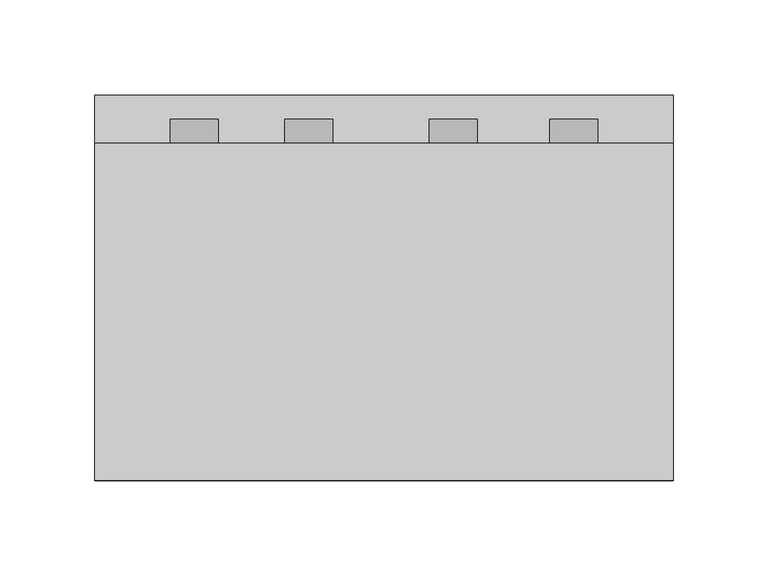
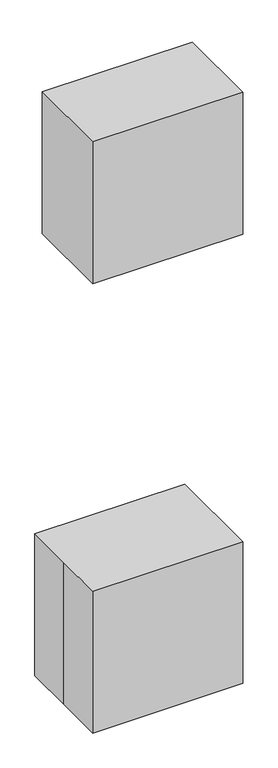
"""IFC4 building model written with IfcOpenShell, lengths in millimetres: proxy geometry, M7845 - Monitor, Physiological, Bedside, 4 Channel-mobile : M7845 - Monitor, Physiological, Bedside, 4 Channel-mobile."""

import ifcopenshell
import ifcopenshell.guid

model = None  # the IFC model being written
_history = None  # IfcOwnerHistory: only IFC2X3 demands one
_inside = {}  # id of a spatial element -> (the spatial element, [elements in it])
_under = {}  # id of a project, library or spatial element -> (it, [spatial elements below it])
_declared = {}  # id of a project -> (the project, [libraries it declares])
_typed = {}  # id of a type object -> (the type object, [elements of that type])
_made_of = {}  # id of a material, layer set ... -> (it, [elements and type objects made of it])


def new_model(schema):
    """Start an empty IFC model of exactly this schema.

    Asked for "IFC4X3", IfcOpenShell would pick the latest addendum, in which some entities
    have other attributes; the version numbers below select the first issue.
    IFC2X3 requires an IfcOwnerHistory on every rooted entity: one is made here for all.
    """
    global model, _history
    if schema == "IFC4X3":
        model = ifcopenshell.file(schema_version=(4, 3, 0, 0))
    else:
        model = ifcopenshell.file(schema=schema)
    _inside.clear()
    _under.clear()
    _declared.clear()
    _typed.clear()
    _made_of.clear()
    _history = None
    if model.schema == "IFC2X3":
        org = make("IfcOrganization", Name="unknown")
        user = make(
            "IfcPersonAndOrganization",
            ThePerson=make("IfcPerson", FamilyName="unknown"),
            TheOrganization=org,
        )
        app = make(
            "IfcApplication",
            ApplicationDeveloper=org,
            Version="unknown",
            ApplicationFullName="unknown",
            ApplicationIdentifier="unknown",
        )
        _history = make(
            "IfcOwnerHistory",
            OwningUser=user,
            OwningApplication=app,
            ChangeAction="ADDED",
            CreationDate=0,
        )
    return model


def make(cls, **values):
    """One entity of the class cls with the attributes given. An attribute that is None is left unset."""
    return model.create_entity(
        cls, **{name: value for name, value in values.items() if value is not None}
    )


def rooted(cls, **values):
    """An entity with a GlobalId (a new one), such as an element, a storey or a relation."""
    return make(cls, GlobalId=ifcopenshell.guid.new(), OwnerHistory=_history, **values)


def si_unit(unit_type, name, prefix=None):
    """IfcSIUnit, for example si_unit("LENGTHUNIT", "METRE", prefix="MILLI")."""
    return make("IfcSIUnit", UnitType=unit_type, Prefix=prefix, Name=name)


def assignment(units):
    """IfcUnitAssignment: the units of a project."""
    return None if units is None else make("IfcUnitAssignment", Units=units)


def point(xyz):
    """IfcCartesianPoint."""
    return None if xyz is None else make("IfcCartesianPoint", Coordinates=xyz)


def direction(xyz):
    """IfcDirection."""
    return None if xyz is None else make("IfcDirection", DirectionRatios=xyz)


def frame(location, z_axis=None, x_axis=None):
    """IfcAxis2Placement3D, a coordinate frame: its origin and axes. An axis left out is left unset."""
    return make(
        "IfcAxis2Placement3D",
        Location=point(location),
        Axis=direction(z_axis),
        RefDirection=direction(x_axis),
    )


def frame_2d(location, x_axis=None):
    """IfcAxis2Placement2D, a coordinate frame in the plane: its origin and x axis."""
    return make(
        "IfcAxis2Placement2D", Location=point(location), RefDirection=direction(x_axis)
    )


def origin():
    """The frame at (0, 0, 0) with its axes left unset."""
    return frame((0.0, 0.0, 0.0))


def origin_with_axes():
    """The frame at (0, 0, 0) with the z axis (0, 0, 1) and the x axis (1, 0, 0) written out."""
    return frame((0.0, 0.0, 0.0), z_axis=(0.0, 0.0, 1.0), x_axis=(1.0, 0.0, 0.0))


def place(relative_to, where):
    """IfcLocalPlacement: puts the frame where relative to a parent placement (None: the world)."""
    return make(
        "IfcLocalPlacement", PlacementRelTo=relative_to, RelativePlacement=where
    )


def context(
    kind, dimensions, precision=None, world=None, true_north=None, identifier=None
):
    """IfcGeometricRepresentationContext, for example the 3D "Model" context."""
    return make(
        "IfcGeometricRepresentationContext",
        ContextIdentifier=identifier,
        ContextType=kind,
        CoordinateSpaceDimension=dimensions,
        Precision=precision,
        WorldCoordinateSystem=world,
        TrueNorth=true_north,
    )


def project(units=None, contexts=None):
    """IfcProject with its units and contexts."""
    return rooted(
        "IfcProject",
        Name="project",
        RepresentationContexts=contexts,
        UnitsInContext=assignment(units),
    )


def spatial(cls, under=None, at=None, **own):
    """A site, building, storey or space (cls), placed at a placement, below another one or the project."""
    s = rooted(cls, ObjectPlacement=at, **own)
    if under is not None:
        _under.setdefault(under.id(), (under, []))[1].append(s)
    return s


def polyline(points):
    """IfcPolyline through the points."""
    return make("IfcPolyline", Points=[point(p) for p in points])


def circle_curve(where, radius):
    """IfcCircle in the frame where."""
    return make("IfcCircle", Position=where, Radius=radius)


def trimmed(basis, trim1, trim2, sense, master):
    """IfcTrimmedCurve: the piece of a basis curve between two trims."""
    return make(
        "IfcTrimmedCurve",
        BasisCurve=basis,
        Trim1=trim1,
        Trim2=trim2,
        SenseAgreement=sense,
        MasterRepresentation=master,
    )


def segment(curve, same_sense, transition):
    """IfcCompositeCurveSegment."""
    return make(
        "IfcCompositeCurveSegment",
        Transition=transition,
        SameSense=same_sense,
        ParentCurve=curve,
    )


def composite_curve(segments, self_intersect=None):
    """IfcCompositeCurve: segments joined end to end."""
    return make("IfcCompositeCurve", Segments=segments, SelfIntersect=self_intersect)


def outline(outer, holes=None, kind="AREA"):
    """IfcArbitraryClosedProfileDef: a profile drawn as a closed curve; with holes, ...WithVoids."""
    if holes is None:
        return make("IfcArbitraryClosedProfileDef", ProfileType=kind, OuterCurve=outer)
    return make(
        "IfcArbitraryProfileDefWithVoids",
        ProfileType=kind,
        OuterCurve=outer,
        InnerCurves=holes,
    )


def extrude(swept, where, along, depth):
    """IfcExtrudedAreaSolid: the profile swept, set in the frame where, extruded along a direction by depth."""
    return make(
        "IfcExtrudedAreaSolid",
        SweptArea=swept,
        Position=where,
        ExtrudedDirection=direction(along),
        Depth=depth,
    )


def faces_of(points, faces, orient=None, outer=None):
    """IfcFace entities. A face is a list of loops; a loop is a list of indices into points, from 0.

    orient and outer hold one flag for each loop. By default every Orientation is true, the
    first loop of a face is its IfcFaceOuterBound and the others are IfcFaceBound.
    """
    made = []
    for i, loops in enumerate(faces):
        bounds = []
        for j, loop in enumerate(loops):
            is_outer = j == 0 if outer is None else outer[i][j]
            bounds.append(
                make(
                    "IfcFaceOuterBound" if is_outer else "IfcFaceBound",
                    Bound=make("IfcPolyLoop", Polygon=[points[k] for k in loop]),
                    Orientation=True if orient is None else orient[i][j],
                )
            )
        made.append(make("IfcFace", Bounds=bounds))
    return made


def faceted_brep(points, faces, orient=None, outer=None, voids=None):
    """IfcFacetedBrep: a solid bounded by flat faces; with voids (closed shells), ...WithVoids."""
    shared = [point(p) for p in points]
    hull = make("IfcClosedShell", CfsFaces=faces_of(shared, faces, orient, outer))
    if voids is None:
        return make("IfcFacetedBrep", Outer=hull)
    return make(
        "IfcFacetedBrepWithVoids",
        Outer=hull,
        Voids=[
            make(cls, CfsFaces=faces_of(shared, fs, o, b)) for cls, fs, o, b in voids
        ],
    )


def shape(context_of_items, identifier, shape_type, items):
    """IfcShapeRepresentation: the items that make up one representation, for example the "Body"."""
    return make(
        "IfcShapeRepresentation",
        ContextOfItems=context_of_items,
        RepresentationIdentifier=identifier,
        RepresentationType=shape_type,
        Items=items,
    )


def source(mapping_origin, context_of_items, identifier, shape_type, items):
    """IfcRepresentationMap: a shape defined once, which mapped items show again and again."""
    return make(
        "IfcRepresentationMap",
        MappingOrigin=mapping_origin,
        MappedRepresentation=shape(context_of_items, identifier, shape_type, items),
    )


def transform(
    local_origin,
    x_axis=None,
    y_axis=None,
    z_axis=None,
    scale=None,
    scale2=None,
    scale3=None,
    uniform=True,
):
    """IfcCartesianTransformationOperator3D, or its non-uniform kind. x_axis, y_axis, z_axis: its Axis1, 2, 3."""
    if uniform:
        return make(
            "IfcCartesianTransformationOperator3D",
            Axis1=direction(x_axis),
            Axis2=direction(y_axis),
            LocalOrigin=point(local_origin),
            Scale=scale,
            Axis3=direction(z_axis),
        )
    return make(
        "IfcCartesianTransformationOperator3DnonUniform",
        Axis1=direction(x_axis),
        Axis2=direction(y_axis),
        LocalOrigin=point(local_origin),
        Scale=scale,
        Axis3=direction(z_axis),
        Scale2=scale2,
        Scale3=scale3,
    )


def mapped(mapping_source, mapping_target):
    """IfcMappedItem: shows the shape of a source again, moved by a transform."""
    return make(
        "IfcMappedItem", MappingSource=mapping_source, MappingTarget=mapping_target
    )


def made_of(thing, what):
    """Note that an element or type object is made of a material, layer set ...; save() writes the relation."""
    if what is not None:
        _made_of.setdefault(what.id(), (what, []))[1].append(thing)
    return thing


def element(
    cls,
    number,
    at=None,
    inside=None,
    cuts=None,
    type_object=None,
    material=None,
    context=None,
    identifier="Body",
    shape_type=None,
    held_by="IfcProductDefinitionShape",
    body=None,
    shapes=None,
    **own,
):
    """One element of the class cls, such as IfcWall. Its Tag is "e" and its number.

    at: its placement. inside: the storey or other place that contains it. cuts: it is an
    opening in that element (IfcRelVoidsElement). A single representation is given by context,
    identifier, shape_type and body (its items); several are given by shapes. held_by: the class
    of the entity that holds the representations. save() writes the other relations.
    """
    e = rooted(cls, Tag="e%d" % number, ObjectPlacement=at, **own)
    if body is not None:
        shapes = [shape(context, identifier, shape_type, body)]
    if shapes is not None:
        e.Representation = make(held_by, Representations=shapes)
    if inside is not None:
        _inside.setdefault(inside.id(), (inside, []))[1].append(e)
    if cuts is not None:
        rooted(
            "IfcRelVoidsElement", RelatingBuildingElement=cuts, RelatedOpeningElement=e
        )
    if type_object is not None:
        _typed.setdefault(type_object.id(), (type_object, []))[1].append(e)
    return made_of(e, material)


def aggregate(whole, parts):
    """IfcRelAggregates: a whole, such as a stair, and the parts it consists of."""
    return rooted("IfcRelAggregates", RelatingObject=whole, RelatedObjects=parts)


def save(model, path):
    """Write the relations noted so far, then the file.

    IfcRelAggregates (storeys below a building ...), IfcRelContainedInSpatialStructure (elements
    in a storey), IfcRelDefinesByType, IfcRelAssociatesMaterial and IfcRelDeclares: one each for
    every whole, place, type object, material and project.
    """
    for whole, parts in _under.values():
        aggregate(whole, parts)
    for where, things in _inside.values():
        rooted(
            "IfcRelContainedInSpatialStructure",
            RelatedElements=things,
            RelatingStructure=where,
        )
    for kind, things in _typed.values():
        rooted("IfcRelDefinesByType", RelatedObjects=things, RelatingType=kind)
    for what, things in _made_of.values():
        rooted("IfcRelAssociatesMaterial", RelatedObjects=things, RelatingMaterial=what)
    for by, libraries in _declared.values():
        rooted("IfcRelDeclares", RelatingContext=by, RelatedDefinitions=libraries)
    model.write(path)


def specialty_equipment_01cb5a5e(model_context):
    return source(origin(), model_context, "Body", "SolidModel", [
        extrude(outline(composite_curve([segment(trimmed(circle_curve(frame_2d((1006.3587525, 100.0366492)), 12.7), [point((1006.3587525, 112.7366492))], [point((1006.3587525, 87.3366492))], False, "CARTESIAN"), True, "CONTINUOUS"), segment(trimmed(circle_curve(frame_2d((1006.3587525, 100.0366492)), 12.7), [point((1006.3587525, 87.3366492))], [point((1006.3587525, 112.7366492))], False, "CARTESIAN"), True, "CONTINUOUS")], self_intersect=False)), frame((0.0, 76.2, 0.0), z_axis=(0.0, 1.0, 0.0), x_axis=(0.0, 0.0, 1.0)), (0.0, 0.0, 1.0), 12.7),
        extrude(outline(composite_curve([segment(trimmed(circle_curve(frame_2d((1006.3587525, -39.7116492)), 12.7), [point((1006.3587525, -52.4116492))], [point((1006.3587525, -27.0116492))], False, "CARTESIAN"), True, "CONTINUOUS"), segment(trimmed(circle_curve(frame_2d((1006.3587525, -39.7116492)), 12.7), [point((1006.3587525, -27.0116492))], [point((1006.3587525, -52.4116492))], False, "CARTESIAN"), True, "CONTINUOUS")], self_intersect=False)), frame((0.0, 76.2, 0.0), z_axis=(0.0, 1.0, 0.0), x_axis=(0.0, 0.0, 1.0)), (0.0, 0.0, 1.0), 12.7),
        extrude(outline(composite_curve([segment(trimmed(circle_curve(frame_2d((1006.3587525, -100.0366492)), 12.7), [point((1006.3587525, -112.7366492))], [point((1006.3587525, -87.3366492))], False, "CARTESIAN"), True, "CONTINUOUS"), segment(trimmed(circle_curve(frame_2d((1006.3587525, -100.0366492)), 12.7), [point((1006.3587525, -87.3366492))], [point((1006.3587525, -112.7366492))], False, "CARTESIAN"), True, "CONTINUOUS")], self_intersect=False)), frame((0.0, 76.2, 0.0), z_axis=(0.0, 1.0, 0.0), x_axis=(0.0, 0.0, 1.0)), (0.0, 0.0, 1.0), 12.7),
        extrude(outline(composite_curve([segment(trimmed(circle_curve(frame_2d((1006.3587525, 36.4883508)), 12.7), [point((1006.3587525, 23.7883508))], [point((1006.3587525, 49.1883508))], False, "CARTESIAN"), True, "CONTINUOUS"), segment(trimmed(circle_curve(frame_2d((1006.3587525, 36.4883508)), 12.7), [point((1006.3587525, 49.1883508))], [point((1006.3587525, 23.7883508))], False, "CARTESIAN"), True, "CONTINUOUS")], self_intersect=False)), frame((0.0, 76.2, 0.0), z_axis=(0.0, 1.0, 0.0), x_axis=(0.0, 0.0, 1.0)), (0.0, 0.0, 1.0), 12.7),
        extrude(outline(polyline([(109.187649, 76.2), (109.187649, 69.85), (-106.712351, 69.85), (-106.712351, 76.2), (109.187649, 76.2)])), frame((0.0, 0.0, 1046.2028485), z_axis=(0.0, 0.0, 1.0), x_axis=(1.0, 0.0, 0.0)), (0.0, 0.0, 1.0), 184.15),
        faceted_brep([(152.4, 76.2, 1270.0), (152.4, 76.2, 965.2), (-152.4, 76.2, 965.2), (-152.4, 76.2, 1270.0), (-106.712351, 76.2, 1230.3528485), (-106.712351, 76.2, 1046.2028485), (109.187649, 76.2, 1046.2028485), (109.187649, 76.2, 1230.3528485), (152.4, -101.6, 1270.0), (-152.4, -101.6, 1270.0), (-152.4, -101.6, 965.2), (152.4, -101.6, 965.2), (109.187649, 63.5, 1230.3528485), (109.187649, 63.5, 1046.2028485), (-106.712351, 63.5, 1046.2028485), (-106.712351, 63.5, 1230.3528485)], [[[0, 1, 2, 3], [4, 5, 6, 7]], [[8, 9, 10, 11]], [[3, 9, 8, 0]], [[2, 10, 9, 3]], [[1, 11, 10, 2]], [[0, 8, 11, 1]], [[12, 13, 14, 15]], [[15, 4, 7, 12]], [[14, 5, 4, 15]], [[13, 6, 5, 14]], [[12, 7, 6, 13]]]),
        extrude(outline(polyline([(-152.4, -101.6), (-152.4, 0.0), (-152.4, 101.6), (152.4, 101.6), (152.4, -101.6), (-152.4, -101.6)])), origin_with_axes(), (0.0, 0.0, 1.0), 304.8),
    ])


if __name__ == "__main__":
    model = new_model("IFC4")
    model_context = context("Model", 3, world=origin())
    ifc_project = project(units=[si_unit("LENGTHUNIT", "METRE", prefix="MILLI")], contexts=[model_context])
    site = spatial("IfcSite", under=ifc_project)
    building = spatial("IfcBuilding", under=site)
    placement = place(None, origin())
    specialty_equipment_shape = specialty_equipment_01cb5a5e(model_context)
    element("IfcBuildingElementProxy", 1, Name="M7845 - Monitor, Physiological, Bedside, 4 Channel-mobile : M7845 - Monitor, Physiological, Bedside, 4 Channel-mobile", ObjectType="M7845 - Monitor, Physiological, Bedside, 4 Channel-mobile : M7845 - Monitor, Physiological, Bedside, 4 Channel-mobile", at=placement, inside=building, context=model_context, shape_type="MappedRepresentation", body=[
        mapped(specialty_equipment_shape, transform((0.0, 0.0, 0.0), x_axis=(1.0, 0.0, 0.0), y_axis=(0.0, 1.0, 0.0), z_axis=(0.0, 0.0, 1.0))),
    ])
    save(model, "model.ifc")

# Revit data of these elements
# Project information
#   Room Abbreviation = "BRMS1/TLTS2"
#   Room Description 2-1 = "Bedroom, Medical/Surgical (BRMS1)"
#   Room Description 2-2 = "Toilet/Shower (TLTS2)"
#   Sheets - Total = "8"
#   Project Issue Date = "Issue Date"
#   Project Status = "Project Status"
#   Client Name = "Owner"
#   Project Address = "Enter address here"
#   Project Name = "Project Name"
#   Project Number = "Project Number"
#   Publication Date = "30-Jan-15"
# Type "M7845 - Monitor, Physiological, Bedside, 4 Channel-mobile : M7845 - Monitor, Physiological, Bedside, 4 Channel-mobile"
#   Watts2 = "0"
#   Watts1 = "360"
#   Unit_Issue = "EA"
#   UTIL_6_Misc = "D"
#   UTIL_5_NonMedGas = "-"
#   UTIL_4_MiscGas = "-"
#   UTIL_3_MedGas = "-"
#   UTIL_2_Elec = "A"
#   UTIL_1_WaterDrain = "-"
#   Nomenclature = "Monitor, Physiological, Bedside, 4 Channel"
#   NSN = "6515"
#   Location [instance default] = ""
#   JSN = "M7845"
#   Fund_Source_VA = "-"
#   Fund_Source_Navy = "-"
#   Fund_Source_Army = "-"
#   Fund_Source_AF = "-"
#   ELEC_Volts2 = "0"
#   ELEC_Volts1 = "120"
#   ELEC_Phase2 = "0"
#   ELEC_Phase1 = "1"
#   ELEC_HertzSwitch = "0"
#   ELEC_HertzDependent = "-1"
#   ELEC_Hertz = "60"
#   ELEC_Amps2 = "0"
#   ELEC_Amps1 = "3"
#   DetailDescription = "4 channel bedside physiological monitor. The unit consist of a four-channel non-fade monochrome display monitor, an alarm system and printer-recording capabilities. The monitor has color coded controls and automatic calibration. The unit displays up to four waveforms simultaneously. The parameters to be monitored are user selectable. The monitor may be connected to a central monitoring station. The unit monitors patients in most acute care areas, step-down units, procedure rooms and emergency rooms."
#   CAT_VA = "C"
#   CAT_Navy = "C"
#   CAT_IHS = "-"
#   CAT_Army = "C"
#   CAT_AF = "C"
#   BTUperhour = "0"
#   Weight_IP = 12
#   DIM_Width_IP = 1' - 0"
#   DIM_Height_IP = 1' - 0"
#   DIM_Depth_IP = 0' - 8"
#   finish [instance default] = none
# Element 1 (IfcBuildingElementProxy, "M7845 - Monitor, Physiological, Bedside, 4 Channel-mobile : M7845 - Monitor, Physiological, Bedside, 4 Channel-mobile")
#   Materials on its faces: "EquipSpace", "Glass"
# Materials
#   "EquipSpace": class "Unassigned", colour RGB 221 217 195, transparency 0.5
#   "Glass": class "Glass", colour RGB 0 128 192, transparency 0.75
